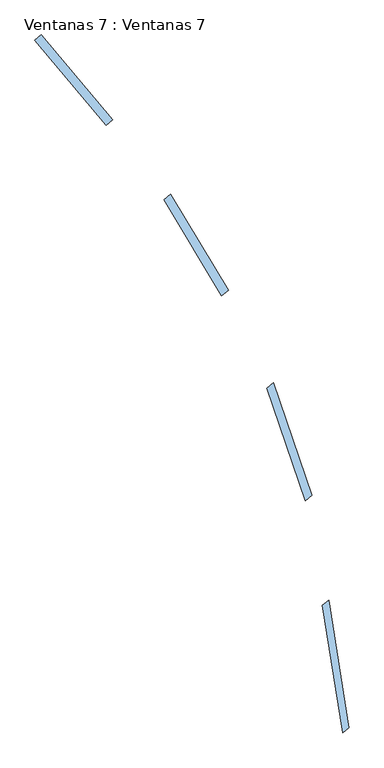
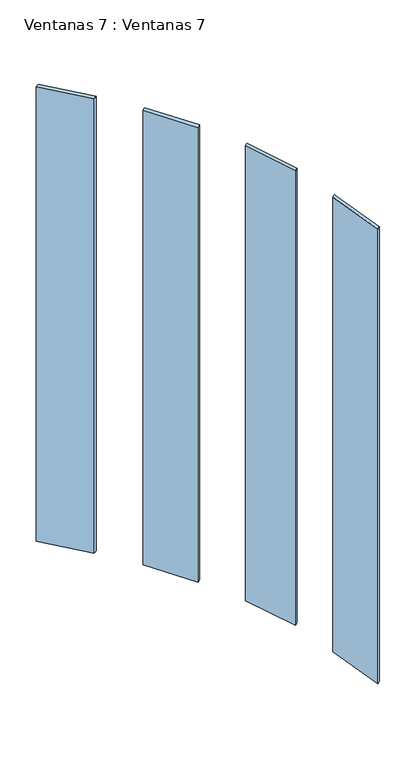
"""IFC4 building model written with IfcOpenShell, lengths in millimetres: window geometry, Ventanas 7 : Ventanas 7."""

from ifc_helpers import new_model, si_unit, frame, origin, place, context, project, spatial, polyline, outline, extrude, source, transform, mapped, element, save


def ventanas_7_ventanas_7_7b9b609b(model_context):
    return source(origin(), model_context, "Body", "SweptSolid", [
        extrude(outline(polyline([(5305.9040786, -93.4413387), (5290.5831897, -106.2970909), (5124.0943714, 92.1165565), (5139.4152603, 104.9723087), (5305.9040786, -93.4413387)])), frame((0.0, 0.0, 5400.0), z_axis=(0.0, 0.0, 1.0), x_axis=(1.0, 0.0, 0.0)), (0.0, 0.0, 1.0), 2327.8129716),
        extrude(outline(polyline([(5577.1048405, -492.4723782), (5561.7839516, -505.3281304), (5426.7207678, -280.5452448), (5442.0416567, -267.6894926), (5577.1048405, -492.4723782)])), frame((0.0, 0.0, 5400.0), z_axis=(0.0, 0.0, 1.0), x_axis=(1.0, 0.0, 0.0)), (0.0, 0.0, 1.0), 2327.8129716),
        extrude(outline(polyline([(5773.220378, -971.6979328), (5757.8994892, -984.553685), (5667.5745341, -722.2309681), (5682.895423, -709.3752159), (5773.220378, -971.6979328)])), frame((0.0, 0.0, 5400.0), z_axis=(0.0, 0.0, 1.0), x_axis=(1.0, 0.0, 0.0)), (0.0, 0.0, 1.0), 2327.8129716),
        extrude(outline(polyline([(5859.412545, -1515.8938575), (5844.952288, -1528.0274538), (5797.6824166, -1229.5772321), (5812.1426736, -1217.4436357), (5859.412545, -1515.8938575)])), frame((0.0, 0.0, 5400.0), z_axis=(0.0, 0.0, 1.0), x_axis=(1.0, 0.0, 0.0)), (0.0, 0.0, 1.0), 2327.8129716),
    ])


if __name__ == "__main__":
    model = new_model("IFC4")
    model_context = context("Model", 3, world=origin())
    ifc_project = project(units=[si_unit("LENGTHUNIT", "METRE", prefix="MILLI")], contexts=[model_context])
    site = spatial("IfcSite", under=ifc_project)
    building = spatial("IfcBuilding", under=site)
    placement = place(None, origin())
    ventanas_7_ventanas_7_shape = ventanas_7_ventanas_7_7b9b609b(model_context)
    element("IfcWindow", 1, ObjectType="Ventanas 7 : Ventanas 7", at=placement, inside=building, context=model_context, shape_type="MappedRepresentation", body=[
        mapped(ventanas_7_ventanas_7_shape, transform((0.0, 0.0, 0.0), x_axis=(1.0, 0.0, 0.0), y_axis=(0.0, 1.0, 0.0), z_axis=(0.0, 0.0, 1.0))),
    ])
    save(model, "model.ifc")

# Revit data of these elements
# Type "Ventanas 7 : Ventanas 7"
#   Type Mark = "33"
# Element 1 (IfcWindow, "Ventanas 7 : Ventanas 7")
#   Materials on its faces: "VIDRIO"
# Materials
#   "VIDRIO": class "Genérico", colour RGB 120 120 120, transparency 0, Cost = 0
